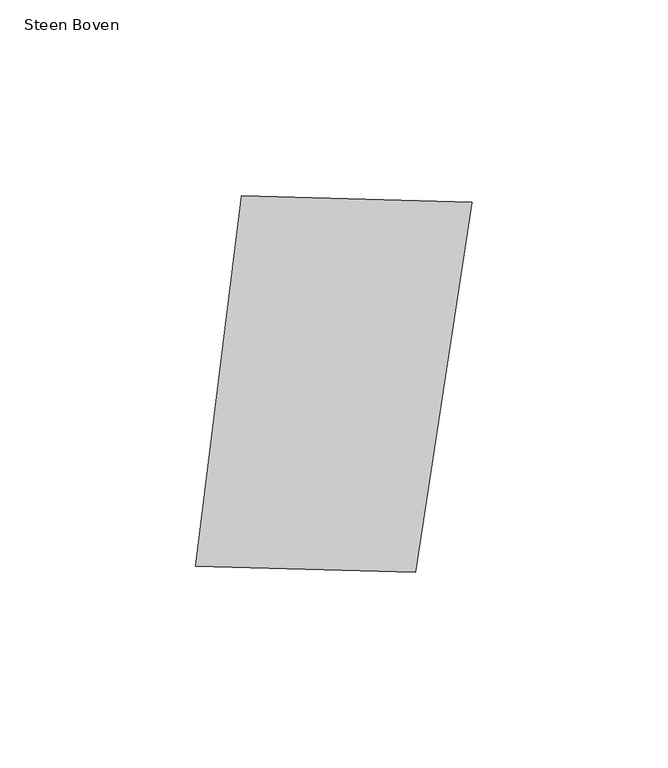
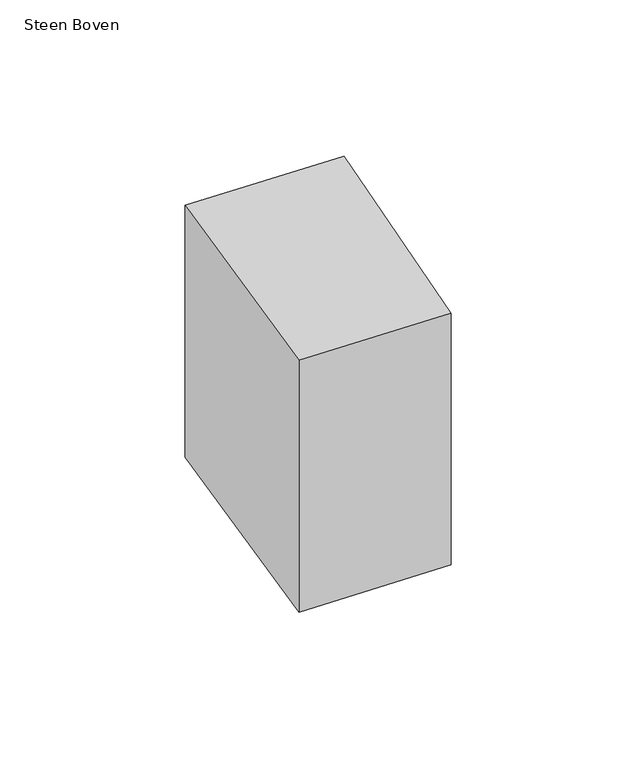
"""IFC4 building model written with IfcOpenShell, lengths in millimetres: proxy geometry, 00_GMA_steen_versie_4 : Steen Boven."""

from ifc_helpers import new_model, si_unit, origin, origin_with_axes, place, context, project, spatial, polyline, outline, extrude, source, transform, mapped, element, save


def steen_boven_4abb9939(model_context):
    return source(origin(), model_context, "Body", "SweptSolid", [
        extrude(outline(polyline([(108.1602922, 118.5428629), (93.704652, 23.8737179), (37.3847868, 25.4648208), (49.2179184, 120.1947689), (108.1602922, 118.5428629)])), origin_with_axes(), (0.0, 0.0, 1.0), 100.0),
    ])


if __name__ == "__main__":
    model = new_model("IFC4")
    model_context = context("Model", 3, world=origin())
    ifc_project = project(units=[si_unit("LENGTHUNIT", "METRE", prefix="MILLI")], contexts=[model_context])
    site = spatial("IfcSite", under=ifc_project)
    building = spatial("IfcBuilding", under=site)
    placement = place(None, origin())
    steen_boven_shape = steen_boven_4abb9939(model_context)
    element("IfcBuildingElementProxy", 1, Name="00_GMA_steen_versie_4 : Steen Boven", ObjectType="00_GMA_steen_versie_4 : Steen Boven", at=placement, inside=building, context=model_context, shape_type="MappedRepresentation", body=[
        mapped(steen_boven_shape, transform((0.0, 0.0, 0.0), x_axis=(1.0, 0.0, 0.0), y_axis=(0.0, 1.0, 0.0), z_axis=(0.0, 0.0, 1.0))),
    ])
    save(model, "model.ifc")

# Revit data of these elements
# Type "00_GMA_steen_versie_4 : Steen Boven"
#   StootVoegHalfBoven [instance default] = 5 mm
#   StootVoegHalf [instance default] = 5 mm
#   StootVoegBreedteOnder = 10 mm
#   StootVoegBreedteBoven = 10 mm
#   Steendikte = 100 mm
#   LintVoegOnderHalf = 5 mm
#   LintVoegOnder = 10 mm
#   LintVoegBovenHalf = 0 mm
#   LintVoegBoven = 0 mm
#   materiaal = none
#   MateriaalVoeg = none
#   Default Elevation = 0
